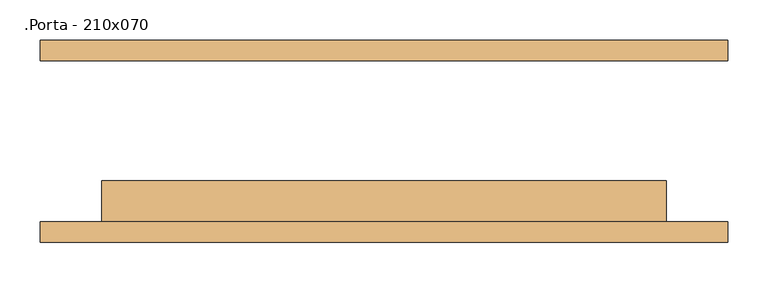
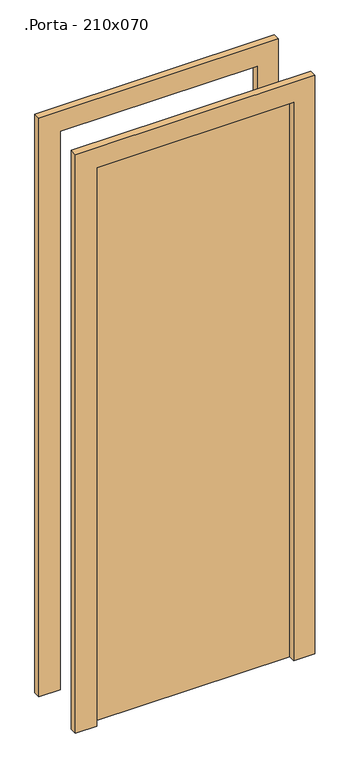
"""IFC4 building model written with IfcOpenShell, lengths in millimetres: door geometry, M_Folha única : .Porta - 210x070."""

from ifc_helpers import new_model, si_unit, frame, origin, origin_with_axes, place, context, project, spatial, polyline, outline, extrude, source, transform, mapped, element, save


def porta_210x070_b827da78(model_context):
    return source(origin(), model_context, "Body", "SweptSolid", [
        extrude(outline(polyline([(2176.0, -426.0), (0.0, -426.0), (0.0, -350.0), (2100.0, -350.0), (2100.0, 350.0), (0.0, 350.0), (0.0, 426.0), (2176.0, 426.0), (2176.0, -426.0)])), frame((0.0, -125.0, 0.0), z_axis=(0.0, 1.0, 0.0), x_axis=(0.0, 0.0, 1.0)), (0.0, 0.0, 1.0), 25.0),
        extrude(outline(polyline([(2176.0, 426.0), (2176.0, -426.0), (0.0, -426.0), (0.0, -350.0), (2100.0, -350.0), (2100.0, 350.0), (0.0, 350.0), (0.0, 426.0), (2176.0, 426.0)])), frame((0.0, 100.0, 0.0), z_axis=(0.0, 1.0, 0.0), x_axis=(0.0, 0.0, 1.0)), (0.0, 0.0, 1.0), 25.0),
        extrude(outline(polyline([(350.0, -49.0), (350.0, -100.0), (-350.0, -100.0), (-350.0, -49.0), (350.0, -49.0)])), origin_with_axes(), (0.0, 0.0, 1.0), 2100.0),
    ])


if __name__ == "__main__":
    model = new_model("IFC4")
    model_context = context("Model", 3, world=origin())
    ifc_project = project(units=[si_unit("LENGTHUNIT", "METRE", prefix="MILLI")], contexts=[model_context])
    site = spatial("IfcSite", under=ifc_project)
    building = spatial("IfcBuilding", under=site)
    placement = place(None, origin())
    porta_210x070_shape = porta_210x070_b827da78(model_context)
    element("IfcDoor", 1, ObjectType="M_Folha única : .Porta - 210x070", at=placement, inside=building, context=model_context, shape_type="MappedRepresentation", body=[
        mapped(porta_210x070_shape, transform((0.0, 0.0, 0.0), x_axis=(1.0, 0.0, 0.0), y_axis=(0.0, 1.0, 0.0), z_axis=(0.0, 0.0, 1.0))),
    ])
    save(model, "model.ifc")

# Revit data of these elements
# Type "M_Folha única : .Porta - 210x070"
#   Type Mark = "40"
#   Construction Type Id = "MDOOR"
#   Analytic Construction = "Metal"
#   Thickness = 0.051 m
#   Thermal Resistance (R) = 0.270117 (m²·K)/W
#   Heat Transfer Coefficient (U) = 3.7021 W/(m²·K)
#   Height = 2.10 m
#   Projeção da apara externa = 0.025 m
#   Projeção da apara interna = 0.025 m
#   Largura da apara = 0.076 m
#   Width = 0.70 m
#   Define Thermal Properties by = 1
#   Material da porta = Porta - Painel
#   Material da moldura = Porta - Batente
#   Visual Light Transmittance = 0
#   Solar Heat Gain Coefficient = 0
#   Function = (empty or 0)
#   Wall Closure = (empty or 0)
# Element 1 (IfcDoor, "M_Folha única : .Porta - 210x070")
#   Materials on its faces: "Porta - Batente", "Porta - Painel"
# Materials
#   "Porta - Painel": class "Madeira", colour RGB 210 159 95, transparency 0, Cost = 0
#   "Porta - Batente": class "Diversos", colour RGB 118 70 51, transparency 0, Cost = 0
